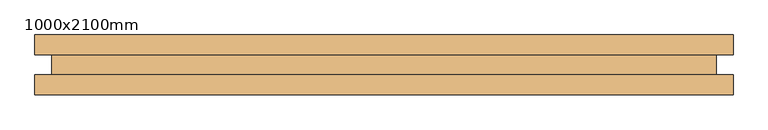
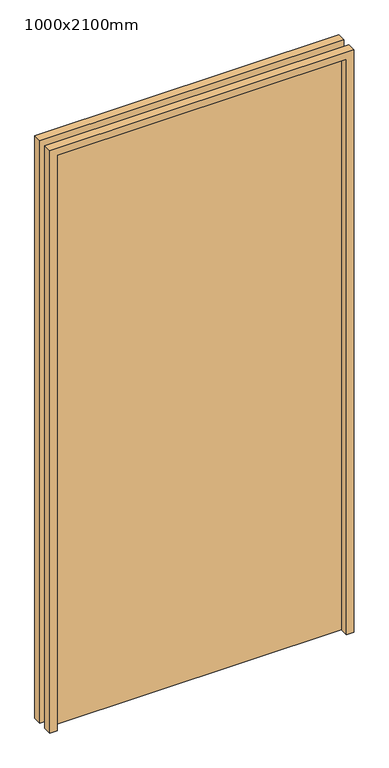
"""IFC4 building model written with IfcOpenShell, lengths in millimetres: door geometry, WWm-SingleSolid-Flush : 1000x2100mm."""

import ifcopenshell
import ifcopenshell.guid

model = None  # the IFC model being written
_history = None  # IfcOwnerHistory: only IFC2X3 demands one
_inside = {}  # id of a spatial element -> (the spatial element, [elements in it])
_under = {}  # id of a project, library or spatial element -> (it, [spatial elements below it])
_declared = {}  # id of a project -> (the project, [libraries it declares])
_typed = {}  # id of a type object -> (the type object, [elements of that type])
_made_of = {}  # id of a material, layer set ... -> (it, [elements and type objects made of it])


def new_model(schema):
    """Start an empty IFC model of exactly this schema.

    Asked for "IFC4X3", IfcOpenShell would pick the latest addendum, in which some entities
    have other attributes; the version numbers below select the first issue.
    IFC2X3 requires an IfcOwnerHistory on every rooted entity: one is made here for all.
    """
    global model, _history
    if schema == "IFC4X3":
        model = ifcopenshell.file(schema_version=(4, 3, 0, 0))
    else:
        model = ifcopenshell.file(schema=schema)
    _inside.clear()
    _under.clear()
    _declared.clear()
    _typed.clear()
    _made_of.clear()
    _history = None
    if model.schema == "IFC2X3":
        org = make("IfcOrganization", Name="unknown")
        user = make(
            "IfcPersonAndOrganization",
            ThePerson=make("IfcPerson", FamilyName="unknown"),
            TheOrganization=org,
        )
        app = make(
            "IfcApplication",
            ApplicationDeveloper=org,
            Version="unknown",
            ApplicationFullName="unknown",
            ApplicationIdentifier="unknown",
        )
        _history = make(
            "IfcOwnerHistory",
            OwningUser=user,
            OwningApplication=app,
            ChangeAction="ADDED",
            CreationDate=0,
        )
    return model


def make(cls, **values):
    """One entity of the class cls with the attributes given. An attribute that is None is left unset."""
    return model.create_entity(
        cls, **{name: value for name, value in values.items() if value is not None}
    )


def rooted(cls, **values):
    """An entity with a GlobalId (a new one), such as an element, a storey or a relation."""
    return make(cls, GlobalId=ifcopenshell.guid.new(), OwnerHistory=_history, **values)


def si_unit(unit_type, name, prefix=None):
    """IfcSIUnit, for example si_unit("LENGTHUNIT", "METRE", prefix="MILLI")."""
    return make("IfcSIUnit", UnitType=unit_type, Prefix=prefix, Name=name)


def assignment(units):
    """IfcUnitAssignment: the units of a project."""
    return None if units is None else make("IfcUnitAssignment", Units=units)


def point(xyz):
    """IfcCartesianPoint."""
    return None if xyz is None else make("IfcCartesianPoint", Coordinates=xyz)


def direction(xyz):
    """IfcDirection."""
    return None if xyz is None else make("IfcDirection", DirectionRatios=xyz)


def frame(location, z_axis=None, x_axis=None):
    """IfcAxis2Placement3D, a coordinate frame: its origin and axes. An axis left out is left unset."""
    return make(
        "IfcAxis2Placement3D",
        Location=point(location),
        Axis=direction(z_axis),
        RefDirection=direction(x_axis),
    )


def origin():
    """The frame at (0, 0, 0) with its axes left unset."""
    return frame((0.0, 0.0, 0.0))


def origin_with_axes():
    """The frame at (0, 0, 0) with the z axis (0, 0, 1) and the x axis (1, 0, 0) written out."""
    return frame((0.0, 0.0, 0.0), z_axis=(0.0, 0.0, 1.0), x_axis=(1.0, 0.0, 0.0))


def place(relative_to, where):
    """IfcLocalPlacement: puts the frame where relative to a parent placement (None: the world)."""
    return make(
        "IfcLocalPlacement", PlacementRelTo=relative_to, RelativePlacement=where
    )


def context(
    kind, dimensions, precision=None, world=None, true_north=None, identifier=None
):
    """IfcGeometricRepresentationContext, for example the 3D "Model" context."""
    return make(
        "IfcGeometricRepresentationContext",
        ContextIdentifier=identifier,
        ContextType=kind,
        CoordinateSpaceDimension=dimensions,
        Precision=precision,
        WorldCoordinateSystem=world,
        TrueNorth=true_north,
    )


def project(units=None, contexts=None):
    """IfcProject with its units and contexts."""
    return rooted(
        "IfcProject",
        Name="project",
        RepresentationContexts=contexts,
        UnitsInContext=assignment(units),
    )


def spatial(cls, under=None, at=None, **own):
    """A site, building, storey or space (cls), placed at a placement, below another one or the project."""
    s = rooted(cls, ObjectPlacement=at, **own)
    if under is not None:
        _under.setdefault(under.id(), (under, []))[1].append(s)
    return s


def polyline(points):
    """IfcPolyline through the points."""
    return make("IfcPolyline", Points=[point(p) for p in points])


def outline(outer, holes=None, kind="AREA"):
    """IfcArbitraryClosedProfileDef: a profile drawn as a closed curve; with holes, ...WithVoids."""
    if holes is None:
        return make("IfcArbitraryClosedProfileDef", ProfileType=kind, OuterCurve=outer)
    return make(
        "IfcArbitraryProfileDefWithVoids",
        ProfileType=kind,
        OuterCurve=outer,
        InnerCurves=holes,
    )


def extrude(swept, where, along, depth):
    """IfcExtrudedAreaSolid: the profile swept, set in the frame where, extruded along a direction by depth."""
    return make(
        "IfcExtrudedAreaSolid",
        SweptArea=swept,
        Position=where,
        ExtrudedDirection=direction(along),
        Depth=depth,
    )


def shape(context_of_items, identifier, shape_type, items):
    """IfcShapeRepresentation: the items that make up one representation, for example the "Body"."""
    return make(
        "IfcShapeRepresentation",
        ContextOfItems=context_of_items,
        RepresentationIdentifier=identifier,
        RepresentationType=shape_type,
        Items=items,
    )


def source(mapping_origin, context_of_items, identifier, shape_type, items):
    """IfcRepresentationMap: a shape defined once, which mapped items show again and again."""
    return make(
        "IfcRepresentationMap",
        MappingOrigin=mapping_origin,
        MappedRepresentation=shape(context_of_items, identifier, shape_type, items),
    )


def transform(
    local_origin,
    x_axis=None,
    y_axis=None,
    z_axis=None,
    scale=None,
    scale2=None,
    scale3=None,
    uniform=True,
):
    """IfcCartesianTransformationOperator3D, or its non-uniform kind. x_axis, y_axis, z_axis: its Axis1, 2, 3."""
    if uniform:
        return make(
            "IfcCartesianTransformationOperator3D",
            Axis1=direction(x_axis),
            Axis2=direction(y_axis),
            LocalOrigin=point(local_origin),
            Scale=scale,
            Axis3=direction(z_axis),
        )
    return make(
        "IfcCartesianTransformationOperator3DnonUniform",
        Axis1=direction(x_axis),
        Axis2=direction(y_axis),
        LocalOrigin=point(local_origin),
        Scale=scale,
        Axis3=direction(z_axis),
        Scale2=scale2,
        Scale3=scale3,
    )


def mapped(mapping_source, mapping_target):
    """IfcMappedItem: shows the shape of a source again, moved by a transform."""
    return make(
        "IfcMappedItem", MappingSource=mapping_source, MappingTarget=mapping_target
    )


def made_of(thing, what):
    """Note that an element or type object is made of a material, layer set ...; save() writes the relation."""
    if what is not None:
        _made_of.setdefault(what.id(), (what, []))[1].append(thing)
    return thing


def element(
    cls,
    number,
    at=None,
    inside=None,
    cuts=None,
    type_object=None,
    material=None,
    context=None,
    identifier="Body",
    shape_type=None,
    held_by="IfcProductDefinitionShape",
    body=None,
    shapes=None,
    **own,
):
    """One element of the class cls, such as IfcWall. Its Tag is "e" and its number.

    at: its placement. inside: the storey or other place that contains it. cuts: it is an
    opening in that element (IfcRelVoidsElement). A single representation is given by context,
    identifier, shape_type and body (its items); several are given by shapes. held_by: the class
    of the entity that holds the representations. save() writes the other relations.
    """
    e = rooted(cls, Tag="e%d" % number, ObjectPlacement=at, **own)
    if body is not None:
        shapes = [shape(context, identifier, shape_type, body)]
    if shapes is not None:
        e.Representation = make(held_by, Representations=shapes)
    if inside is not None:
        _inside.setdefault(inside.id(), (inside, []))[1].append(e)
    if cuts is not None:
        rooted(
            "IfcRelVoidsElement", RelatingBuildingElement=cuts, RelatedOpeningElement=e
        )
    if type_object is not None:
        _typed.setdefault(type_object.id(), (type_object, []))[1].append(e)
    return made_of(e, material)


def aggregate(whole, parts):
    """IfcRelAggregates: a whole, such as a stair, and the parts it consists of."""
    return rooted("IfcRelAggregates", RelatingObject=whole, RelatedObjects=parts)


def save(model, path):
    """Write the relations noted so far, then the file.

    IfcRelAggregates (storeys below a building ...), IfcRelContainedInSpatialStructure (elements
    in a storey), IfcRelDefinesByType, IfcRelAssociatesMaterial and IfcRelDeclares: one each for
    every whole, place, type object, material and project.
    """
    for whole, parts in _under.values():
        aggregate(whole, parts)
    for where, things in _inside.values():
        rooted(
            "IfcRelContainedInSpatialStructure",
            RelatedElements=things,
            RelatingStructure=where,
        )
    for kind, things in _typed.values():
        rooted("IfcRelDefinesByType", RelatedObjects=things, RelatingType=kind)
    for what, things in _made_of.values():
        rooted("IfcRelAssociatesMaterial", RelatedObjects=things, RelatingMaterial=what)
    for by, libraries in _declared.values():
        rooted("IfcRelDeclares", RelatingContext=by, RelatedDefinitions=libraries)
    model.write(path)


def door_1000x2100mm_85672f94(model_context):
    return source(origin(), model_context, "Body", "SweptSolid", [
        extrude(outline(polyline([(2125.0, -525.0), (0.0, -525.0), (0.0, -500.0), (2100.0, -500.0), (2100.0, 500.0), (0.0, 500.0), (0.0, 525.0), (2125.0, 525.0), (2125.0, -525.0)])), frame((0.0, -45.0, 0.0), z_axis=(0.0, 1.0, 0.0), x_axis=(0.0, 0.0, 1.0)), (0.0, 0.0, 1.0), 30.0),
        extrude(outline(polyline([(2125.0, 525.0), (2125.0, -525.0), (0.0, -525.0), (0.0, -500.0), (2100.0, -500.0), (2100.0, 500.0), (0.0, 500.0), (0.0, 525.0), (2125.0, 525.0)])), frame((0.0, 15.0, 0.0), z_axis=(0.0, 1.0, 0.0), x_axis=(0.0, 0.0, 1.0)), (0.0, 0.0, 1.0), 30.0),
        extrude(outline(polyline([(500.0, 35.0), (500.0, -15.0), (-500.0, -15.0), (-500.0, 35.0), (500.0, 35.0)])), origin_with_axes(), (0.0, 0.0, 1.0), 2100.0),
    ])


if __name__ == "__main__":
    model = new_model("IFC4")
    model_context = context("Model", 3, world=origin())
    ifc_project = project(units=[si_unit("LENGTHUNIT", "METRE", prefix="MILLI")], contexts=[model_context])
    site = spatial("IfcSite", under=ifc_project)
    building = spatial("IfcBuilding", under=site)
    placement = place(None, origin())
    door_1000x2100mm_shape = door_1000x2100mm_85672f94(model_context)
    element("IfcDoor", 1, ObjectType="WWm-SingleSolid-Flush : 1000x2100mm", at=placement, inside=building, context=model_context, shape_type="MappedRepresentation", body=[
        mapped(door_1000x2100mm_shape, transform((0.0, 0.0, 0.0), x_axis=(1.0, 0.0, 0.0), y_axis=(0.0, 1.0, 0.0), z_axis=(0.0, 0.0, 1.0))),
    ])
    save(model, "model.ifc")

# Revit data of these elements
# Type "WWm-SingleSolid-Flush : 1000x2100mm"
#   Type Mark = "EX1-51"
#   Construction Type Id = "MDOOR"
#   Assembly Code = "C1020"
#   Analytic Construction = "Metal"
#   Thickness = 50 mm
#   Thermal Resistance (R) = 0.270117 (m²·K)/W
#   Heat Transfer Coefficient (U) = 3.7021 W/(m²·K)
#   Height = 2100 mm
#   Trim Projection Ext = 30 mm
#   Trim Projection Int = 30 mm
#   Trim Width = 25 mm
#   Width = 1000 mm
#   Not 90 Degree [instance default] = no
#   90 Degree [instance default] = yes
#   Door Material = WW-EC-RGB-White
#   Frame Material = WW-EC-RGB-White
#   Visual Light Transmittance = 0
#   Solar Heat Gain Coefficient = 0
#   Function = (empty or 0)
#   Wall Closure = (empty or 0)
# Element 1 (IfcDoor, "WWm-SingleSolid-Flush : 1000x2100mm")
#   Materials on its faces: "WW-EC-RGB-White"
# Materials
#   "WW-EC-RGB-White": class "Generic", colour RGB 255 255 255, transparency 0, Comments = "If region requests off-white, swith asset color to RGB 231-228-220", Description = "Generic Color", Cost = 0
